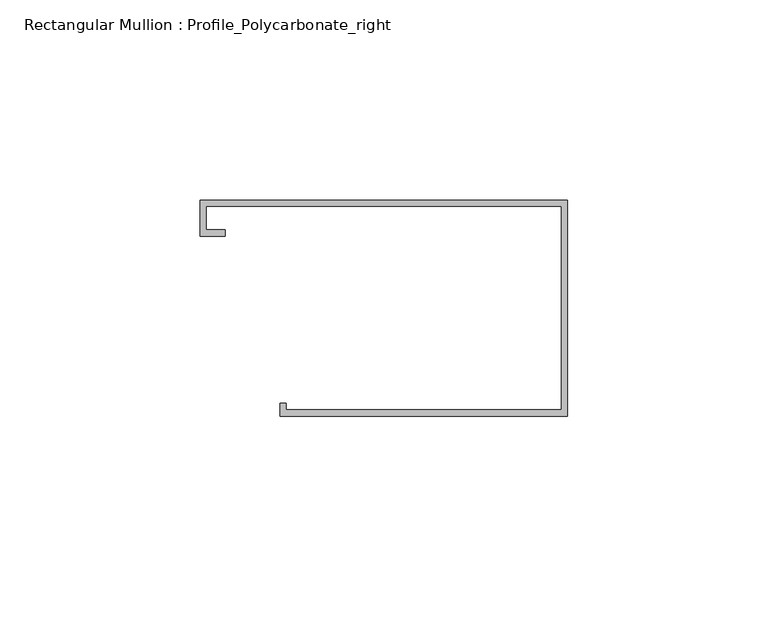
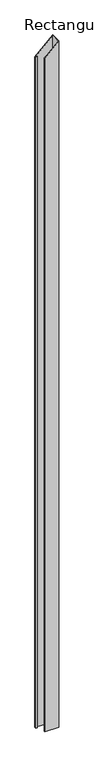
"""IFC4 building model written with IfcOpenShell, lengths in millimetres: member geometry, Rectangular Mullion : Profile_Polycarbonate_right."""

from ifc_helpers import new_model, si_unit, origin, place, context, project, spatial, faceted_brep, source, transform, mapped, element, save


def rectangular_mullion_profile_polycarbonate_right_d47f4ab6(model_context):
    return source(origin(), model_context, "Body", "Brep", [
        faceted_brep([(0.0, 28.984575, -3762.1928295), (0.0, -25.015825, -3762.1928295), (-71.9836, -25.015825, -3762.1928295), (-71.9836, -21.840825, -3762.1928295), (-70.3961, -21.840825, -3762.1928295), (-70.3961, -23.428325, -3762.1928295), (-1.5875, -23.428325, -3762.1928295), (-1.5875, 27.397075, -3762.1928295), (-90.4113, 27.397075, -3762.1928295), (-90.4113, 21.580475, -3762.1928295), (-85.6488, 21.580475, -3762.1928295), (-85.6488, 19.992975, -3762.1928295), (-91.9988, 19.992975, -3762.1928295), (-91.9988, 28.984575, -3762.1928295), (-91.9988, 28.984575, -88.2453421), (0.0, 28.984575, 0.0), (-91.9988, 19.992975, -88.2453421), (-85.6488, 19.992975, -82.1544157), (-85.6488, 21.580475, -82.1544157), (-90.4113, 21.580475, -86.7226105), (-90.4113, 27.397075, -86.7226105), (-1.5875, 27.397075, -1.5227316), (-1.5875, -23.428325, -1.5227316), (-70.3961, -23.428325, -67.5240104), (-70.3961, -21.840825, -67.5240104), (-71.9836, -21.840825, -69.046742), (-71.9836, -25.015825, -69.046742), (0.0, -25.015825, 0.0)], [[[0, 1, 2, 3, 4, 5, 6, 7, 8, 9, 10, 11, 12, 13]], [[14, 15, 0, 13]], [[16, 14, 13, 12]], [[17, 16, 12, 11]], [[18, 17, 11, 10]], [[19, 18, 10, 9]], [[20, 19, 9, 8]], [[21, 20, 8, 7]], [[22, 21, 7, 6]], [[23, 22, 6, 5]], [[24, 23, 5, 4]], [[25, 24, 4, 3]], [[26, 25, 3, 2]], [[27, 26, 2, 1]], [[15, 27, 1, 0]], [[15, 14, 16, 17, 18, 19, 20, 21, 22, 23, 24, 25, 26, 27]]]),
    ])


if __name__ == "__main__":
    model = new_model("IFC4")
    model_context = context("Model", 3, world=origin())
    ifc_project = project(units=[si_unit("LENGTHUNIT", "METRE", prefix="MILLI")], contexts=[model_context])
    site = spatial("IfcSite", under=ifc_project)
    building = spatial("IfcBuilding", under=site)
    placement = place(None, origin())
    rectangular_mullion_profile_polycarbonate_right_shape = rectangular_mullion_profile_polycarbonate_right_d47f4ab6(model_context)
    element("IfcMember", 1, ObjectType="Rectangular Mullion : Profile_Polycarbonate_right", at=placement, inside=building, context=model_context, shape_type="MappedRepresentation", body=[
        mapped(rectangular_mullion_profile_polycarbonate_right_shape, transform((0.0, 0.0, 0.0), x_axis=(1.0, 0.0, 0.0), y_axis=(0.0, 1.0, 0.0), z_axis=(0.0, 0.0, 1.0))),
    ])
    save(model, "model.ifc")

# Revit data of these elements
# Type "Rectangular Mullion : Profile_Polycarbonate_right"
#   built-in parameter 1007322 = 0.177167 (stored number, unit not read)
#   built-in parameter 1007321 = 0 (stored number, unit not read)
#   built-in parameter 1007320 = 0.00520833 (stored number, unit not read)
